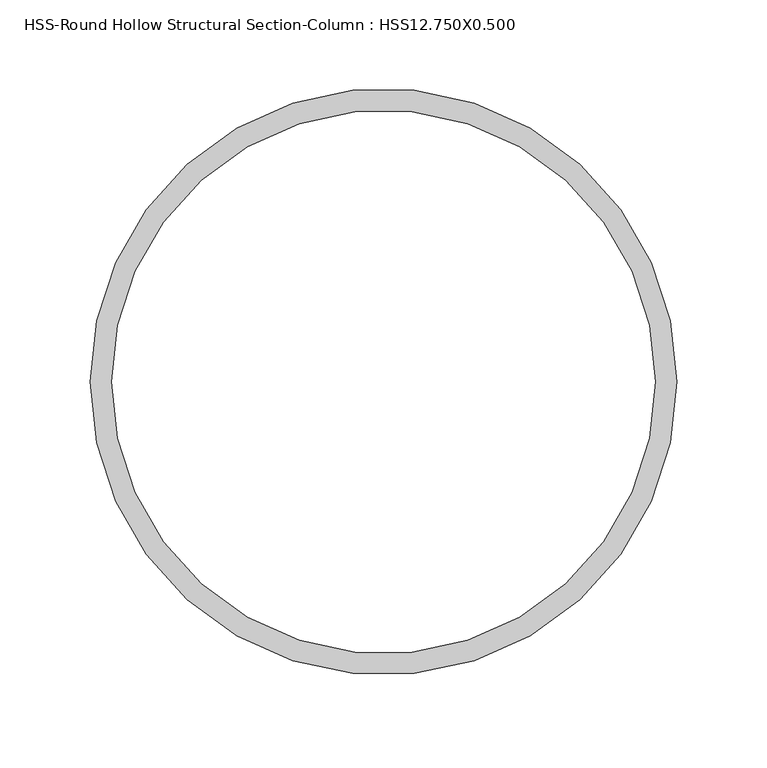
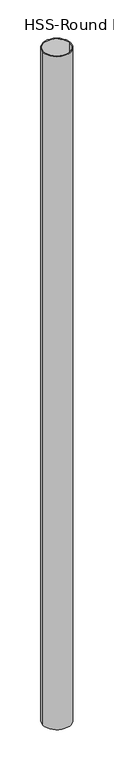
"""IFC4 building model written with IfcOpenShell, lengths in millimetres: column geometry, HSS-Round Hollow Structural Section-Column : HSS12.750X0.500."""

from ifc_helpers import new_model, si_unit, point, frame, origin, origin_2d, place, context, project, spatial, circle_curve, trimmed, segment, composite_curve, outline, extrude, source, transform, mapped, element, save


def hss_round_hollow_structural_section_column_hss12_750x0_500_ca34f2c9(model_context):
    return source(origin(), model_context, "Body", "SweptSolid", [
        extrude(outline(composite_curve([segment(trimmed(circle_curve(origin_2d(), 161.925), [point((-161.925, 0.0))], [point((161.925, 0.0))], False, "CARTESIAN"), True, "CONTINUOUS"), segment(trimmed(circle_curve(origin_2d(), 161.925), [point((161.925, 0.0))], [point((-161.925, 0.0))], False, "CARTESIAN"), True, "CONTINUOUS")], self_intersect=False), holes=[composite_curve([segment(trimmed(circle_curve(origin_2d(), 150.114), [point((-150.114, 0.0))], [point((150.114, 0.0))], True, "CARTESIAN"), True, "CONTINUOUS"), segment(trimmed(circle_curve(origin_2d(), 150.114), [point((150.114, 0.0))], [point((-150.114, 0.0))], True, "CARTESIAN"), True, "CONTINUOUS")], self_intersect=False)]), frame((0.0, 0.0, 12065.0), z_axis=(0.0, 0.0, 1.0), x_axis=(1.0, 0.0, 0.0)), (0.0, 0.0, 1.0), 8280.4),
    ])


if __name__ == "__main__":
    model = new_model("IFC4")
    model_context = context("Model", 3, world=origin())
    ifc_project = project(units=[si_unit("LENGTHUNIT", "METRE", prefix="MILLI")], contexts=[model_context])
    site = spatial("IfcSite", under=ifc_project)
    building = spatial("IfcBuilding", under=site)
    placement = place(None, origin())
    hss_round_hollow_structural_section_column_hss12_750x0_500_shape = hss_round_hollow_structural_section_column_hss12_750x0_500_ca34f2c9(model_context)
    element("IfcColumn", 1, ObjectType="HSS-Round Hollow Structural Section-Column : HSS12.750X0.500", at=placement, inside=building, context=model_context, shape_type="MappedRepresentation", body=[
        mapped(hss_round_hollow_structural_section_column_hss12_750x0_500_shape, transform((0.0, 0.0, 0.0), x_axis=(1.0, 0.0, 0.0), y_axis=(0.0, 1.0, 0.0), z_axis=(0.0, 0.0, 1.0))),
    ])
    save(model, "model.ifc")

# Revit data of these elements
# Type "HSS-Round Hollow Structural Section-Column : HSS12.750X0.500"
#   Assembly Code = "B10"
#   W = 65.5
#   OD = 1' - 0 3/4"
#   t = 0' - 0.465"
#   A = 0.124306 SF
#   Column Material [instance default] = Metal - Steel - ASTM A53
# Element 1 (IfcColumn, "HSS-Round Hollow Structural Section-Column : HSS12.750X0.500")
#   Materials on its faces: "Metal - Steel - ASTM A53"
# Materials
#   "Metal - Steel - ASTM A53": class "Metal", colour RGB 128 0 0, transparency 0
